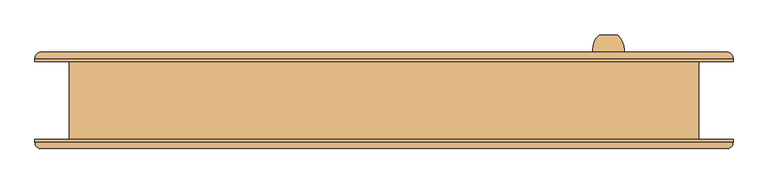
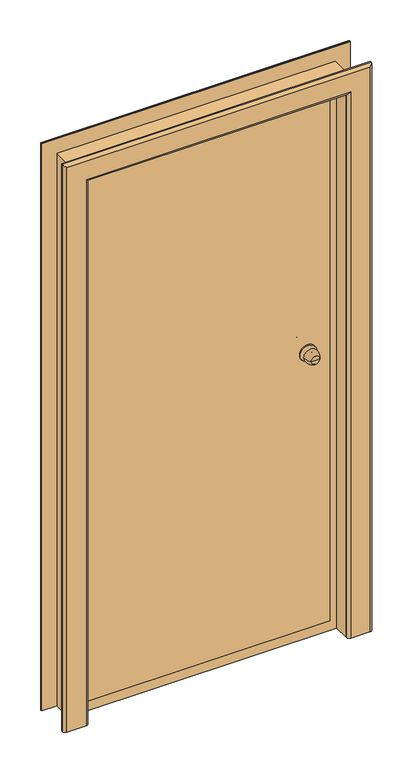
"""IFC4 building model written with IfcOpenShell, lengths in millimetres: door geometry, Наружная дверь 1-Навесная - Один проем наружу с порогом - 31173-2003 : ДСН КЛН  М1 УЗ 2100-1010 ГОСТ 31173-2003."""

import ifcopenshell
import ifcopenshell.guid

model = None  # the IFC model being written
_history = None  # IfcOwnerHistory: only IFC2X3 demands one
_inside = {}  # id of a spatial element -> (the spatial element, [elements in it])
_under = {}  # id of a project, library or spatial element -> (it, [spatial elements below it])
_declared = {}  # id of a project -> (the project, [libraries it declares])
_typed = {}  # id of a type object -> (the type object, [elements of that type])
_made_of = {}  # id of a material, layer set ... -> (it, [elements and type objects made of it])


def new_model(schema):
    """Start an empty IFC model of exactly this schema.

    Asked for "IFC4X3", IfcOpenShell would pick the latest addendum, in which some entities
    have other attributes; the version numbers below select the first issue.
    IFC2X3 requires an IfcOwnerHistory on every rooted entity: one is made here for all.
    """
    global model, _history
    if schema == "IFC4X3":
        model = ifcopenshell.file(schema_version=(4, 3, 0, 0))
    else:
        model = ifcopenshell.file(schema=schema)
    _inside.clear()
    _under.clear()
    _declared.clear()
    _typed.clear()
    _made_of.clear()
    _history = None
    if model.schema == "IFC2X3":
        org = make("IfcOrganization", Name="unknown")
        user = make(
            "IfcPersonAndOrganization",
            ThePerson=make("IfcPerson", FamilyName="unknown"),
            TheOrganization=org,
        )
        app = make(
            "IfcApplication",
            ApplicationDeveloper=org,
            Version="unknown",
            ApplicationFullName="unknown",
            ApplicationIdentifier="unknown",
        )
        _history = make(
            "IfcOwnerHistory",
            OwningUser=user,
            OwningApplication=app,
            ChangeAction="ADDED",
            CreationDate=0,
        )
    return model


def make(cls, **values):
    """One entity of the class cls with the attributes given. An attribute that is None is left unset."""
    return model.create_entity(
        cls, **{name: value for name, value in values.items() if value is not None}
    )


def rooted(cls, **values):
    """An entity with a GlobalId (a new one), such as an element, a storey or a relation."""
    return make(cls, GlobalId=ifcopenshell.guid.new(), OwnerHistory=_history, **values)


def si_unit(unit_type, name, prefix=None):
    """IfcSIUnit, for example si_unit("LENGTHUNIT", "METRE", prefix="MILLI")."""
    return make("IfcSIUnit", UnitType=unit_type, Prefix=prefix, Name=name)


def assignment(units):
    """IfcUnitAssignment: the units of a project."""
    return None if units is None else make("IfcUnitAssignment", Units=units)


def point(xyz):
    """IfcCartesianPoint."""
    return None if xyz is None else make("IfcCartesianPoint", Coordinates=xyz)


def direction(xyz):
    """IfcDirection."""
    return None if xyz is None else make("IfcDirection", DirectionRatios=xyz)


def frame(location, z_axis=None, x_axis=None):
    """IfcAxis2Placement3D, a coordinate frame: its origin and axes. An axis left out is left unset."""
    return make(
        "IfcAxis2Placement3D",
        Location=point(location),
        Axis=direction(z_axis),
        RefDirection=direction(x_axis),
    )


def origin():
    """The frame at (0, 0, 0) with its axes left unset."""
    return frame((0.0, 0.0, 0.0))


def place(relative_to, where):
    """IfcLocalPlacement: puts the frame where relative to a parent placement (None: the world)."""
    return make(
        "IfcLocalPlacement", PlacementRelTo=relative_to, RelativePlacement=where
    )


def context(
    kind, dimensions, precision=None, world=None, true_north=None, identifier=None
):
    """IfcGeometricRepresentationContext, for example the 3D "Model" context."""
    return make(
        "IfcGeometricRepresentationContext",
        ContextIdentifier=identifier,
        ContextType=kind,
        CoordinateSpaceDimension=dimensions,
        Precision=precision,
        WorldCoordinateSystem=world,
        TrueNorth=true_north,
    )


def project(units=None, contexts=None):
    """IfcProject with its units and contexts."""
    return rooted(
        "IfcProject",
        Name="project",
        RepresentationContexts=contexts,
        UnitsInContext=assignment(units),
    )


def spatial(cls, under=None, at=None, **own):
    """A site, building, storey or space (cls), placed at a placement, below another one or the project."""
    s = rooted(cls, ObjectPlacement=at, **own)
    if under is not None:
        _under.setdefault(under.id(), (under, []))[1].append(s)
    return s


def polyline(points):
    """IfcPolyline through the points."""
    return make("IfcPolyline", Points=[point(p) for p in points])


def circle_curve(where, radius):
    """IfcCircle in the frame where."""
    return make("IfcCircle", Position=where, Radius=radius)


def ellipse_curve(where, semi_axis1, semi_axis2):
    """IfcEllipse in the frame where."""
    return make(
        "IfcEllipse", Position=where, SemiAxis1=semi_axis1, SemiAxis2=semi_axis2
    )


def trimmed(basis, trim1, trim2, sense, master):
    """IfcTrimmedCurve: the piece of a basis curve between two trims."""
    return make(
        "IfcTrimmedCurve",
        BasisCurve=basis,
        Trim1=trim1,
        Trim2=trim2,
        SenseAgreement=sense,
        MasterRepresentation=master,
    )


def outline(outer, holes=None, kind="AREA"):
    """IfcArbitraryClosedProfileDef: a profile drawn as a closed curve; with holes, ...WithVoids."""
    if holes is None:
        return make("IfcArbitraryClosedProfileDef", ProfileType=kind, OuterCurve=outer)
    return make(
        "IfcArbitraryProfileDefWithVoids",
        ProfileType=kind,
        OuterCurve=outer,
        InnerCurves=holes,
    )


def extrude(swept, where, along, depth):
    """IfcExtrudedAreaSolid: the profile swept, set in the frame where, extruded along a direction by depth."""
    return make(
        "IfcExtrudedAreaSolid",
        SweptArea=swept,
        Position=where,
        ExtrudedDirection=direction(along),
        Depth=depth,
    )


def faces_of(points, faces, orient=None, outer=None):
    """IfcFace entities. A face is a list of loops; a loop is a list of indices into points, from 0.

    orient and outer hold one flag for each loop. By default every Orientation is true, the
    first loop of a face is its IfcFaceOuterBound and the others are IfcFaceBound.
    """
    made = []
    for i, loops in enumerate(faces):
        bounds = []
        for j, loop in enumerate(loops):
            is_outer = j == 0 if outer is None else outer[i][j]
            bounds.append(
                make(
                    "IfcFaceOuterBound" if is_outer else "IfcFaceBound",
                    Bound=make("IfcPolyLoop", Polygon=[points[k] for k in loop]),
                    Orientation=True if orient is None else orient[i][j],
                )
            )
        made.append(make("IfcFace", Bounds=bounds))
    return made


def faceted_brep(points, faces, orient=None, outer=None, voids=None):
    """IfcFacetedBrep: a solid bounded by flat faces; with voids (closed shells), ...WithVoids."""
    shared = [point(p) for p in points]
    hull = make("IfcClosedShell", CfsFaces=faces_of(shared, faces, orient, outer))
    if voids is None:
        return make("IfcFacetedBrep", Outer=hull)
    return make(
        "IfcFacetedBrepWithVoids",
        Outer=hull,
        Voids=[
            make(cls, CfsFaces=faces_of(shared, fs, o, b)) for cls, fs, o, b in voids
        ],
    )


def shape(context_of_items, identifier, shape_type, items):
    """IfcShapeRepresentation: the items that make up one representation, for example the "Body"."""
    return make(
        "IfcShapeRepresentation",
        ContextOfItems=context_of_items,
        RepresentationIdentifier=identifier,
        RepresentationType=shape_type,
        Items=items,
    )


def source(mapping_origin, context_of_items, identifier, shape_type, items):
    """IfcRepresentationMap: a shape defined once, which mapped items show again and again."""
    return make(
        "IfcRepresentationMap",
        MappingOrigin=mapping_origin,
        MappedRepresentation=shape(context_of_items, identifier, shape_type, items),
    )


def transform(
    local_origin,
    x_axis=None,
    y_axis=None,
    z_axis=None,
    scale=None,
    scale2=None,
    scale3=None,
    uniform=True,
):
    """IfcCartesianTransformationOperator3D, or its non-uniform kind. x_axis, y_axis, z_axis: its Axis1, 2, 3."""
    if uniform:
        return make(
            "IfcCartesianTransformationOperator3D",
            Axis1=direction(x_axis),
            Axis2=direction(y_axis),
            LocalOrigin=point(local_origin),
            Scale=scale,
            Axis3=direction(z_axis),
        )
    return make(
        "IfcCartesianTransformationOperator3DnonUniform",
        Axis1=direction(x_axis),
        Axis2=direction(y_axis),
        LocalOrigin=point(local_origin),
        Scale=scale,
        Axis3=direction(z_axis),
        Scale2=scale2,
        Scale3=scale3,
    )


def mapped(mapping_source, mapping_target):
    """IfcMappedItem: shows the shape of a source again, moved by a transform."""
    return make(
        "IfcMappedItem", MappingSource=mapping_source, MappingTarget=mapping_target
    )


def made_of(thing, what):
    """Note that an element or type object is made of a material, layer set ...; save() writes the relation."""
    if what is not None:
        _made_of.setdefault(what.id(), (what, []))[1].append(thing)
    return thing


def element(
    cls,
    number,
    at=None,
    inside=None,
    cuts=None,
    type_object=None,
    material=None,
    context=None,
    identifier="Body",
    shape_type=None,
    held_by="IfcProductDefinitionShape",
    body=None,
    shapes=None,
    **own,
):
    """One element of the class cls, such as IfcWall. Its Tag is "e" and its number.

    at: its placement. inside: the storey or other place that contains it. cuts: it is an
    opening in that element (IfcRelVoidsElement). A single representation is given by context,
    identifier, shape_type and body (its items); several are given by shapes. held_by: the class
    of the entity that holds the representations. save() writes the other relations.
    """
    e = rooted(cls, Tag="e%d" % number, ObjectPlacement=at, **own)
    if body is not None:
        shapes = [shape(context, identifier, shape_type, body)]
    if shapes is not None:
        e.Representation = make(held_by, Representations=shapes)
    if inside is not None:
        _inside.setdefault(inside.id(), (inside, []))[1].append(e)
    if cuts is not None:
        rooted(
            "IfcRelVoidsElement", RelatingBuildingElement=cuts, RelatedOpeningElement=e
        )
    if type_object is not None:
        _typed.setdefault(type_object.id(), (type_object, []))[1].append(e)
    return made_of(e, material)


def aggregate(whole, parts):
    """IfcRelAggregates: a whole, such as a stair, and the parts it consists of."""
    return rooted("IfcRelAggregates", RelatingObject=whole, RelatedObjects=parts)


def save(model, path):
    """Write the relations noted so far, then the file.

    IfcRelAggregates (storeys below a building ...), IfcRelContainedInSpatialStructure (elements
    in a storey), IfcRelDefinesByType, IfcRelAssociatesMaterial and IfcRelDeclares: one each for
    every whole, place, type object, material and project.
    """
    for whole, parts in _under.values():
        aggregate(whole, parts)
    for where, things in _inside.values():
        rooted(
            "IfcRelContainedInSpatialStructure",
            RelatedElements=things,
            RelatingStructure=where,
        )
    for kind, things in _typed.values():
        rooted("IfcRelDefinesByType", RelatedObjects=things, RelatingType=kind)
    for what, things in _made_of.values():
        rooted("IfcRelAssociatesMaterial", RelatedObjects=things, RelatingMaterial=what)
    for by, libraries in _declared.values():
        rooted("IfcRelDeclares", RelatingContext=by, RelatedDefinitions=libraries)
    model.write(path)


def plane_surface(at):
    """IfcPlane: the flat surface through the origin of the frame at, square to its z axis."""
    return make("IfcPlane", Position=at)


def cylinder_surface(at, radius):
    """IfcCylindricalSurface: all points at the distance radius from the z axis of the frame at."""
    return make("IfcCylindricalSurface", Position=at, Radius=radius)


def revolved_surface(curve, axis_point, axis_direction):
    """IfcSurfaceOfRevolution: the curve turned about the line through axis_point along axis_direction."""
    return make(
        "IfcSurfaceOfRevolution",
        SweptCurve=make("IfcArbitraryOpenProfileDef", ProfileType="CURVE", Curve=curve),
        AxisPosition=make("IfcAxis1Placement", Location=point(axis_point), Axis=direction(axis_direction)),
    )


def advanced_brep(points, edges, surfaces, faces):
    """IfcAdvancedBrep: a solid bounded by faces that lie on surfaces and meet in shared edges.

    An edge is (start, end): straight between two places in points (the first is 0);
    or (start, end, curve); or (start, end, curve, False) where it runs against its curve.
    A face is (place in surfaces, loops), or (place, loops, False) where it looks against
    its surface's normal. A loop lists edges by number (the first is 1), with a minus sign
    where the edge is run from its end to its start. The first loop is the outer one.
    """
    corners = [point(p) for p in points]
    vertices = [make("IfcVertexPoint", VertexGeometry=c) for c in corners]
    made = []
    for start, end, *more in edges:
        made.append(
            make(
                "IfcEdgeCurve",
                EdgeStart=vertices[start],
                EdgeEnd=vertices[end],
                EdgeGeometry=more[0] if more else make("IfcPolyline", Points=[corners[start], corners[end]]),
                SameSense=more[1] if len(more) > 1 else True,
            )
        )
    hull = []
    for where, loops, *sense in faces:
        bounds = []
        for j, loop in enumerate(loops):
            ring = [make("IfcOrientedEdge", EdgeElement=made[abs(k) - 1], Orientation=k > 0) for k in loop]
            bounds.append(
                make(
                    "IfcFaceOuterBound" if j == 0 else "IfcFaceBound",
                    Bound=make("IfcEdgeLoop", EdgeList=ring),
                    Orientation=True,
                )
            )
        hull.append(make("IfcAdvancedFace", Bounds=bounds, FaceSurface=surfaces[where], SameSense=sense[0] if sense else True))
    return make("IfcAdvancedBrep", Outer=make("IfcClosedShell", CfsFaces=hull))


def door_5ac3ea5e(model_context):
    return source(origin(), model_context, "Body", "SolidModel", [
        advanced_brep(
        [(345.0, 105.5, 1100.0), (375.0, 105.5, 1100.0), (360.0, 105.5, 1100.0), (335.0, 75.5, 1100.0), (385.0, 75.5, 1100.0), (342.0, 75.5, 1100.0), (378.0, 75.5, 1100.0), (350.0, 67.5, 1100.0), (370.0, 67.5, 1100.0), (350.0, 61.5, 1100.0), (370.0, 61.5, 1100.0), (390.0, 61.5, 1100.0), (330.0, 61.5, 1100.0), (390.0, 55.5, 1100.0), (330.0, 55.5, 1100.0)],
        [
            (0, 1, circle_curve(frame((360.0, 105.5, 1100.0), z_axis=(0.0, 1.0, 0.0), x_axis=(1.0, 0.0, 0.0)), 15.0)),
            (1, 2),
            (2, 0),
            (1, 0, circle_curve(frame((360.0, 105.5, 1100.0), z_axis=(0.0, 1.0, 0.0), x_axis=(1.0, 0.0, 0.0)), 15.0)),
            (0, 3, circle_curve(frame((369.6226265, 80.6257912, 1100.0), z_axis=(0.0, 0.0, 1.0), x_axis=(1.0, 0.0, 0.0)), 35.0)),
            (3, 4, circle_curve(frame((360.0, 75.5, 1100.0), z_axis=(0.0, 1.0, 0.0), x_axis=(1.0, 0.0, 0.0)), 25.0)),
            (4, 1, circle_curve(frame((350.3773735, 80.6257912, 1100.0), z_axis=(0.0, 0.0, 1.0), x_axis=(-1.0, 0.0, 0.0)), 35.0)),
            (4, 3, circle_curve(frame((360.0, 75.5, 1100.0), z_axis=(0.0, 1.0, 0.0), x_axis=(1.0, 0.0, 0.0)), 25.0)),
            (3, 5),
            (5, 6, circle_curve(frame((360.0, 75.5, 1100.0), z_axis=(0.0, 1.0, 0.0), x_axis=(1.0, 0.0, 0.0)), 18.0)),
            (6, 4),
            (6, 5, circle_curve(frame((360.0, 75.5, 1100.0), z_axis=(0.0, 1.0, 0.0), x_axis=(1.0, 0.0, 0.0)), 18.0)),
            (5, 7, circle_curve(frame((342.0, 67.5, 1100.0), z_axis=(0.0, 0.0, -1.0), x_axis=(1.0, 0.0, 0.0)), 8.0)),
            (7, 8, circle_curve(frame((360.0, 67.5, 1100.0), z_axis=(0.0, 1.0, 0.0), x_axis=(1.0, 0.0, 0.0)), 10.0)),
            (8, 6, circle_curve(frame((378.0, 67.5, 1100.0), z_axis=(0.0, 0.0, -1.0), x_axis=(-1.0, 0.0, 0.0)), 8.0)),
            (8, 7, circle_curve(frame((360.0, 67.5, 1100.0), z_axis=(0.0, 1.0, 0.0), x_axis=(1.0, 0.0, 0.0)), 10.0)),
            (7, 9),
            (9, 10, circle_curve(frame((360.0, 61.5, 1100.0), z_axis=(0.0, 1.0, 0.0), x_axis=(1.0, 0.0, 0.0)), 10.0)),
            (10, 8),
            (10, 9, circle_curve(frame((360.0, 61.5, 1100.0), z_axis=(0.0, 1.0, 0.0), x_axis=(1.0, 0.0, 0.0)), 10.0)),
            (11, 12, circle_curve(frame((360.0, 61.5, 1100.0), z_axis=(0.0, 1.0, 0.0), x_axis=(-1.0, 0.0, 0.0)), 30.0)),
            (12, 11, circle_curve(frame((360.0, 61.5, 1100.0), z_axis=(0.0, 1.0, 0.0), x_axis=(-1.0, 0.0, 0.0)), 30.0)),
            (13, 14, circle_curve(frame((360.0, 55.5, 1100.0), z_axis=(0.0, -1.0, 0.0), x_axis=(-1.0, 0.0, 0.0)), 30.0)),
            (14, 13, circle_curve(frame((360.0, 55.5, 1100.0), z_axis=(0.0, -1.0, 0.0), x_axis=(-1.0, 0.0, 0.0)), 30.0)),
            (11, 13),
            (14, 12),
        ],
        [
            plane_surface(frame((360.0, 105.5, 1100.0), z_axis=(0.0, 1.0, 0.0), x_axis=(1.0, 0.0, 0.0))),
            revolved_surface(trimmed(ellipse_curve(frame((350.3773735, 80.6257912, 1100.0), z_axis=(0.0, 0.0, -1.0), x_axis=(-1.0, 0.0, 0.0)), 35.0, 35.0), [point((375.0, 105.5, 1100.0))], [point((385.0, 75.5, 1100.0))], True, "CARTESIAN"), (360.0, 135.5, 1100.0), (0.0, -1.0, 0.0)),
            plane_surface(frame((360.0, 75.5, 1100.0), z_axis=(0.0, -1.0, 0.0), x_axis=(1.0, 0.0, 0.0))),
            revolved_surface(trimmed(ellipse_curve(frame((378.0, 67.5, 1100.0), z_axis=(0.0, 0.0, 1.0), x_axis=(-1.0, 0.0, 0.0)), 8.0, 8.0), [point((378.0, 75.5, 1100.0))], [point((370.0, 67.5, 1100.0))], True, "CARTESIAN"), (360.0, 135.5, 1100.0), (0.0, -1.0, 0.0)),
            cylinder_surface(frame((360.0, 135.5, 1100.0), z_axis=(0.0, -1.0, 0.0), x_axis=(1.0, 0.0, 0.0)), 10.0),
            plane_surface(frame((330.0, 61.5, 1100.0), z_axis=(0.0, 1.0, 0.0), x_axis=(0.0, 0.0, 1.0))),
            plane_surface(frame((330.0, 55.5, 1100.0), z_axis=(0.0, -1.0, 0.0), x_axis=(0.0, 0.0, -1.0))),
            cylinder_surface(frame((360.0, 55.5, 1100.0), z_axis=(0.0, 1.0, 0.0), x_axis=(-1.0, 0.0, 0.0)), 30.0),
        ],
        [
            (0, [[1, 2, 3]]),
            (0, [[-2, 4, -3]]),
            (1, [[-1, 5, 6, 7]]),
            (1, [[-4, -7, 8, -5]]),
            (2, [[-6, 9, 10, 11]]),
            (2, [[-8, -11, 12, -9]]),
            (3, [[-10, 13, 14, 15]]),
            (3, [[-12, -15, 16, -13]]),
            (4, [[-14, 17, 18, 19]]),
            (4, [[-16, -19, 20, -17]]),
            (5, [[21, 22], [-18, -20]]),
            (6, [[23, 24]]),
            (7, [[-21, 25, -24, 26]]),
            (7, [[-22, -26, -23, -25]]),
        ],
    ),
        advanced_brep(
        [(375.0, -64.5, 1100.0), (345.0, -64.5, 1100.0), (360.0, -64.5, 1100.0), (385.0, -34.5, 1100.0), (335.0, -34.5, 1100.0), (378.0, -34.5, 1100.0), (342.0, -34.5, 1100.0), (370.0, -26.5, 1100.0), (350.0, -26.5, 1100.0), (370.0, -20.5, 1100.0), (350.0, -20.5, 1100.0), (330.0, -20.5, 1100.0), (390.0, -20.5, 1100.0), (330.0, -14.5, 1100.0), (390.0, -14.5, 1100.0)],
        [
            (0, 1, circle_curve(frame((360.0, -64.5, 1100.0), z_axis=(0.0, -1.0, 0.0), x_axis=(-1.0, 0.0, 0.0)), 15.0)),
            (1, 2),
            (2, 0),
            (1, 0, circle_curve(frame((360.0, -64.5, 1100.0), z_axis=(0.0, -1.0, 0.0), x_axis=(-1.0, 0.0, 0.0)), 15.0)),
            (0, 3, circle_curve(frame((350.3773735, -39.6257912, 1100.0), z_axis=(0.0, 0.0, 1.0), x_axis=(-1.0, 0.0, 0.0)), 35.0)),
            (3, 4, circle_curve(frame((360.0, -34.5, 1100.0), z_axis=(0.0, -1.0, 0.0), x_axis=(-1.0, 0.0, 0.0)), 25.0)),
            (4, 1, circle_curve(frame((369.6226265, -39.6257912, 1100.0), z_axis=(0.0, 0.0, 1.0), x_axis=(1.0, 0.0, 0.0)), 35.0)),
            (4, 3, circle_curve(frame((360.0, -34.5, 1100.0), z_axis=(0.0, -1.0, 0.0), x_axis=(-1.0, 0.0, 0.0)), 25.0)),
            (3, 5),
            (5, 6, circle_curve(frame((360.0, -34.5, 1100.0), z_axis=(0.0, -1.0, 0.0), x_axis=(-1.0, 0.0, 0.0)), 18.0)),
            (6, 4),
            (6, 5, circle_curve(frame((360.0, -34.5, 1100.0), z_axis=(0.0, -1.0, 0.0), x_axis=(-1.0, 0.0, 0.0)), 18.0)),
            (5, 7, circle_curve(frame((378.0, -26.5, 1100.0), z_axis=(0.0, 0.0, -1.0), x_axis=(-1.0, 0.0, 0.0)), 8.0)),
            (7, 8, circle_curve(frame((360.0, -26.5, 1100.0), z_axis=(0.0, -1.0, 0.0), x_axis=(-1.0, 0.0, 0.0)), 10.0)),
            (8, 6, circle_curve(frame((342.0, -26.5, 1100.0), z_axis=(0.0, 0.0, -1.0), x_axis=(1.0, 0.0, 0.0)), 8.0)),
            (8, 7, circle_curve(frame((360.0, -26.5, 1100.0), z_axis=(0.0, -1.0, 0.0), x_axis=(-1.0, 0.0, 0.0)), 10.0)),
            (7, 9),
            (9, 10, circle_curve(frame((360.0, -20.5, 1100.0), z_axis=(0.0, -1.0, 0.0), x_axis=(-1.0, 0.0, 0.0)), 10.0)),
            (10, 8),
            (10, 9, circle_curve(frame((360.0, -20.5, 1100.0), z_axis=(0.0, -1.0, 0.0), x_axis=(-1.0, 0.0, 0.0)), 10.0)),
            (11, 12, circle_curve(frame((360.0, -20.5, 1100.0), z_axis=(0.0, -1.0, 0.0), x_axis=(1.0, 0.0, 0.0)), 30.0)),
            (12, 11, circle_curve(frame((360.0, -20.5, 1100.0), z_axis=(0.0, -1.0, 0.0), x_axis=(1.0, 0.0, 0.0)), 30.0)),
            (13, 14, circle_curve(frame((360.0, -14.5, 1100.0), z_axis=(0.0, 1.0, 0.0), x_axis=(1.0, 0.0, 0.0)), 30.0)),
            (14, 13, circle_curve(frame((360.0, -14.5, 1100.0), z_axis=(0.0, 1.0, 0.0), x_axis=(1.0, 0.0, 0.0)), 30.0)),
            (11, 13),
            (14, 12),
        ],
        [
            plane_surface(frame((360.0, -64.5, 1100.0), z_axis=(0.0, -1.0, 0.0), x_axis=(-1.0, 0.0, 0.0))),
            revolved_surface(trimmed(ellipse_curve(frame((369.6226265, -39.6257912, 1100.0), z_axis=(0.0, 0.0, -1.0), x_axis=(1.0, 0.0, 0.0)), 35.0, 35.0), [point((345.0, -64.5, 1100.0))], [point((335.0, -34.5, 1100.0))], True, "CARTESIAN"), (360.0, -94.5, 1100.0), (0.0, 1.0, 0.0)),
            plane_surface(frame((360.0, -34.5, 1100.0), z_axis=(0.0, 1.0, 0.0), x_axis=(-1.0, 0.0, 0.0))),
            revolved_surface(trimmed(ellipse_curve(frame((342.0, -26.5, 1100.0), z_axis=(0.0, 0.0, 1.0), x_axis=(1.0, 0.0, 0.0)), 8.0, 8.0), [point((342.0, -34.5, 1100.0))], [point((350.0, -26.5, 1100.0))], True, "CARTESIAN"), (360.0, -94.5, 1100.0), (0.0, 1.0, 0.0)),
            cylinder_surface(frame((360.0, -94.5, 1100.0), z_axis=(0.0, 1.0, 0.0), x_axis=(-1.0, 0.0, 0.0)), 10.0),
            plane_surface(frame((390.0, -20.5, 1100.0), z_axis=(0.0, -1.0, 0.0), x_axis=(0.0, 0.0, 1.0))),
            plane_surface(frame((390.0, -14.5, 1100.0), z_axis=(0.0, 1.0, 0.0), x_axis=(0.0, 0.0, -1.0))),
            cylinder_surface(frame((360.0, -14.5, 1100.0), z_axis=(0.0, -1.0, 0.0), x_axis=(1.0, 0.0, 0.0)), 30.0),
        ],
        [
            (0, [[1, 2, 3]]),
            (0, [[-2, 4, -3]]),
            (1, [[-1, 5, 6, 7]]),
            (1, [[-4, -7, 8, -5]]),
            (2, [[-6, 9, 10, 11]]),
            (2, [[-8, -11, 12, -9]]),
            (3, [[-10, 13, 14, 15]]),
            (3, [[-12, -15, 16, -13]]),
            (4, [[-14, 17, 18, 19]]),
            (4, [[-16, -19, 20, -17]]),
            (5, [[21, 22], [-18, -20]]),
            (6, [[23, 24]]),
            (7, [[-21, 25, -24, 26]]),
            (7, [[-22, -26, -23, -25]]),
        ],
    ),
        faceted_brep([(440.0, -14.5, 42.0), (-440.0, -14.5, 42.0), (-440.0, -9.5, 42.0), (440.0, -9.5, 42.0), (440.0, -14.5, 2055.0), (440.0, -9.5, 2055.0), (-440.0, -9.5, 2055.0), (420.0, -9.5, 2035.0), (-420.0, -9.5, 2035.0), (-420.0, -9.5, 62.0), (420.0, -9.5, 62.0), (-440.0, -14.5, 2055.0), (420.0, 55.5, 62.0), (420.0, 55.5, 2035.0), (-420.0, 55.5, 62.0), (-420.0, 55.5, 2035.0)], [[[0, 1, 2, 3]], [[4, 0, 3, 5]], [[5, 3, 2, 6], [7, 8, 9, 10]], [[2, 1, 11, 6]], [[11, 1, 0, 4]], [[7, 10, 12, 13]], [[9, 14, 12, 10]], [[15, 14, 9, 8]], [[13, 12, 14, 15]], [[4, 5, 6, 11]], [[7, 13, 15, 8]]]),
        extrude(outline(polyline([(0.0, 485.0), (2100.0, 485.0), (2100.0, -485.0), (0.0, -485.0), (0.0, -470.0), (2085.0, -470.0), (2085.0, 470.0), (0.0, 470.0), (0.0, 485.0)])), frame((0.0, -62.5, 0.0), z_axis=(0.0, 1.0, 0.0), x_axis=(0.0, 0.0, 1.0)), (0.0, 0.0, 1.0), 55.0),
        faceted_brep([(485.0, -7.5, 0.0), (-485.0, -7.5, 0.0), (-485.0, 62.5, 0.0), (485.0, 62.5, 0.0), (-485.0, -7.5, 2100.0), (-485.0, 62.5, 2100.0), (485.0, 62.5, 2100.0), (-405.0, 62.5, 2020.0), (-405.0, 62.5, 80.0), (405.0, 62.5, 80.0), (405.0, 62.5, 2020.0), (485.0, -7.5, 2100.0), (-425.0, -7.5, 60.0), (-425.0, -7.5, 2040.0), (425.0, -7.5, 2040.0), (425.0, -7.5, 60.0), (425.0, 57.5, 60.0), (-425.0, 57.5, 60.0), (-425.0, 57.5, 2040.0), (425.0, 57.5, 2040.0), (-405.0, 57.5, 80.0), (-405.0, 57.5, 2020.0), (405.0, 57.5, 2020.0), (405.0, 57.5, 80.0)], [[[0, 1, 2, 3]], [[1, 4, 5, 2]], [[2, 5, 6, 3], [7, 8, 9, 10]], [[4, 1, 0, 11], [12, 13, 14, 15]], [[16, 17, 12, 15]], [[17, 18, 13, 12]], [[18, 17, 16, 19], [20, 21, 22, 23]], [[9, 8, 20, 23]], [[8, 7, 21, 20]], [[11, 0, 3, 6]], [[19, 16, 15, 14]], [[10, 9, 23, 22]], [[4, 11, 6, 5]], [[18, 19, 14, 13]], [[7, 10, 22, 21]]]),
        advanced_brep(
        [(-560.0, 62.5, 0.0), (-560.0, 67.5, 0.0), (-550.0, 77.5, 0.0), (-480.0, 77.5, 0.0), (-470.0, 67.5, 0.0), (-470.0, 62.5, 0.0), (-470.0, 62.5, 2085.0), (470.0, 62.5, 2085.0), (470.0, 62.5, 0.0), (560.0, 62.5, 0.0), (560.0, 62.5, 2175.0), (-560.0, 62.5, 2175.0), (-470.0, 67.5, 2085.0), (-480.0, 77.5, 2095.0), (-550.0, 77.5, 2165.0), (550.0, 77.5, 2165.0), (550.0, 77.5, 0.0), (480.0, 77.5, 0.0), (480.0, 77.5, 2095.0), (-560.0, 67.5, 2175.0), (560.0, 67.5, 0.0), (560.0, 67.5, 2175.0), (470.0, 67.5, 0.0), (470.0, 67.5, 2085.0)],
        [
            (0, 1),
            (1, 2, circle_curve(frame((-550.0, 67.5, 0.0), z_axis=(0.0, 0.0, -1.0), x_axis=(-1.0, 0.0, 0.0)), 10.0)),
            (2, 3),
            (3, 4, circle_curve(frame((-480.0, 67.5, 0.0), z_axis=(0.0, 0.0, -1.0), x_axis=(-1.0, 0.0, 0.0)), 10.0)),
            (4, 5),
            (5, 0),
            (5, 6),
            (6, 7),
            (7, 8),
            (8, 9),
            (9, 10),
            (10, 11),
            (11, 0),
            (4, 12),
            (12, 6),
            (3, 13),
            (13, 12, ellipse_curve(frame((-480.0, 67.5, 2095.0), z_axis=(-0.7071067811865475, 0.0, -0.7071067811865475), x_axis=(0.7071067811865474, 0.0, -0.7071067811865476)), 14.1421356, 10.0)),
            (2, 14),
            (14, 15),
            (15, 16),
            (16, 17),
            (17, 18),
            (18, 13),
            (1, 19),
            (19, 14, ellipse_curve(frame((-550.0, 67.5, 2165.0), z_axis=(-0.7071067811865475, 0.0, -0.7071067811865475), x_axis=(0.7071067811865474, 0.0, -0.7071067811865476)), 14.1421356, 10.0)),
            (11, 19),
            (9, 20),
            (20, 21),
            (21, 10),
            (8, 22),
            (22, 17, circle_curve(frame((480.0, 67.5, 0.0), z_axis=(0.0, 0.0, -1.0), x_axis=(1.0, 0.0, 0.0)), 10.0)),
            (16, 20, circle_curve(frame((550.0, 67.5, 0.0), z_axis=(0.0, 0.0, -1.0), x_axis=(1.0, 0.0, 0.0)), 10.0)),
            (23, 22),
            (7, 23),
            (23, 18, ellipse_curve(frame((480.0, 67.5, 2095.0), z_axis=(0.7071067811865475, 0.0, -0.7071067811865475), x_axis=(0.7071067811865474, 0.0, 0.7071067811865476)), 14.1421356, 10.0)),
            (15, 21, ellipse_curve(frame((550.0, 67.5, 2165.0), z_axis=(0.7071067811865475, 0.0, -0.7071067811865475), x_axis=(0.7071067811865474, 0.0, 0.7071067811865476)), 14.1421356, 10.0)),
            (12, 23),
            (19, 21),
        ],
        [
            plane_surface(frame((-505.0, 62.5, 0.0), z_axis=(0.0, 0.0, -1.0), x_axis=(0.0, 1.0, 0.0))),
            plane_surface(frame((-560.0, 62.5, 0.0), z_axis=(0.0, -1.0, 0.0), x_axis=(0.0, 0.0, 1.0))),
            plane_surface(frame((-470.0, 62.5, 0.0), z_axis=(1.0, 0.0, 0.0), x_axis=(0.0, 0.0, 1.0))),
            cylinder_surface(frame((-480.0, 67.5, 0.0), z_axis=(0.0, 0.0, -1.0), x_axis=(-1.0, 0.0, 0.0)), 10.0),
            plane_surface(frame((-480.0, 77.5, 0.0), z_axis=(0.0, 1.0, 0.0), x_axis=(0.0, 0.0, 1.0))),
            cylinder_surface(frame((-550.0, 67.5, 0.0), z_axis=(0.0, 0.0, -1.0), x_axis=(-1.0, 0.0, 0.0)), 10.0),
            plane_surface(frame((-560.0, 67.5, 0.0), z_axis=(-1.0, 0.0, 0.0), x_axis=(0.0, 0.0, 1.0))),
            plane_surface(frame((560.0, 67.5, 2175.0), z_axis=(1.0, 0.0, 0.0), x_axis=(0.0, 0.0, -1.0))),
            plane_surface(frame((505.0, 62.5, 0.0), z_axis=(0.0, 0.0, -1.0), x_axis=(0.0, 1.0, 0.0))),
            plane_surface(frame((470.0, 62.5, 2085.0), z_axis=(-1.0, 0.0, 0.0), x_axis=(0.0, 0.0, -1.0))),
            cylinder_surface(frame((480.0, 67.5, 2120.0), z_axis=(0.0, 0.0, 1.0), x_axis=(1.0, 0.0, 0.0)), 10.0),
            cylinder_surface(frame((550.0, 67.5, 2120.0), z_axis=(0.0, 0.0, 1.0), x_axis=(1.0, 0.0, 0.0)), 10.0),
            plane_surface(frame((-470.0, 62.5, 2085.0), z_axis=(0.0, 0.0, -1.0), x_axis=(1.0, 0.0, 0.0))),
            cylinder_surface(frame((-505.0, 67.5, 2095.0), z_axis=(-1.0, 0.0, 0.0), x_axis=(0.0, 0.0, 1.0)), 10.0),
            cylinder_surface(frame((-505.0, 67.5, 2165.0), z_axis=(-1.0, 0.0, 0.0), x_axis=(0.0, 0.0, 1.0)), 10.0),
            plane_surface(frame((-560.0, 67.5, 2175.0), z_axis=(0.0, 0.0, 1.0), x_axis=(1.0, 0.0, 0.0))),
        ],
        [
            (0, [[1, 2, 3, 4, 5, 6]]),
            (1, [[7, 8, 9, 10, 11, 12, 13, -6]]),
            (2, [[14, 15, -7, -5]]),
            (3, [[16, 17, -14, -4]]),
            (4, [[18, 19, 20, 21, 22, 23, -16, -3]]),
            (5, [[24, 25, -18, -2]]),
            (6, [[-13, 26, -24, -1]]),
            (7, [[-11, 27, 28, 29]]),
            (8, [[-10, 30, 31, -21, 32, -27]]),
            (9, [[33, -30, -9, 34]]),
            (10, [[-22, -31, -33, 35]]),
            (11, [[-28, -32, -20, 36]]),
            (12, [[37, -34, -8, -15]]),
            (13, [[-23, -35, -37, -17]]),
            (14, [[38, -36, -19, -25]]),
            (15, [[-12, -29, -38, -26]]),
        ],
    ),
        advanced_brep(
        [(560.0, -62.5, 0.0), (560.0, -67.5, 0.0), (550.0, -77.5, 0.0), (480.0, -77.5, 0.0), (470.0, -67.5, 0.0), (470.0, -62.5, 0.0), (470.0, -62.5, 2085.0), (-470.0, -62.5, 2085.0), (-470.0, -62.5, 0.0), (-560.0, -62.5, 0.0), (-560.0, -62.5, 2175.0), (560.0, -62.5, 2175.0), (470.0, -67.5, 2085.0), (480.0, -77.5, 2095.0), (550.0, -77.5, 2165.0), (-550.0, -77.5, 2165.0), (-550.0, -77.5, 0.0), (-480.0, -77.5, 0.0), (-480.0, -77.5, 2095.0), (560.0, -67.5, 2175.0), (-560.0, -67.5, 0.0), (-560.0, -67.5, 2175.0), (-470.0, -67.5, 0.0), (-470.0, -67.5, 2085.0)],
        [
            (0, 1),
            (1, 2, circle_curve(frame((550.0, -67.5, 0.0), z_axis=(0.0, 0.0, -1.0), x_axis=(1.0, 0.0, 0.0)), 10.0)),
            (2, 3),
            (3, 4, circle_curve(frame((480.0, -67.5, 0.0), z_axis=(0.0, 0.0, -1.0), x_axis=(1.0, 0.0, 0.0)), 10.0)),
            (4, 5),
            (5, 0),
            (5, 6),
            (6, 7),
            (7, 8),
            (8, 9),
            (9, 10),
            (10, 11),
            (11, 0),
            (4, 12),
            (12, 6),
            (3, 13),
            (13, 12, ellipse_curve(frame((480.0, -67.5, 2095.0), z_axis=(0.7071067811865475, 0.0, -0.7071067811865475), x_axis=(-0.7071067811865474, 0.0, -0.7071067811865476)), 14.1421356, 10.0)),
            (2, 14),
            (14, 15),
            (15, 16),
            (16, 17),
            (17, 18),
            (18, 13),
            (1, 19),
            (19, 14, ellipse_curve(frame((550.0, -67.5, 2165.0), z_axis=(0.7071067811865475, 0.0, -0.7071067811865475), x_axis=(-0.7071067811865474, 0.0, -0.7071067811865476)), 14.1421356, 10.0)),
            (11, 19),
            (9, 20),
            (20, 21),
            (21, 10),
            (8, 22),
            (22, 17, circle_curve(frame((-480.0, -67.5, 0.0), z_axis=(0.0, 0.0, -1.0), x_axis=(-1.0, 0.0, 0.0)), 10.0)),
            (16, 20, circle_curve(frame((-550.0, -67.5, 0.0), z_axis=(0.0, 0.0, -1.0), x_axis=(-1.0, 0.0, 0.0)), 10.0)),
            (23, 22),
            (7, 23),
            (23, 18, ellipse_curve(frame((-480.0, -67.5, 2095.0), z_axis=(-0.7071067811865475, 0.0, -0.7071067811865475), x_axis=(-0.7071067811865474, 0.0, 0.7071067811865476)), 14.1421356, 10.0)),
            (15, 21, ellipse_curve(frame((-550.0, -67.5, 2165.0), z_axis=(-0.7071067811865475, 0.0, -0.7071067811865475), x_axis=(-0.7071067811865474, 0.0, 0.7071067811865476)), 14.1421356, 10.0)),
            (12, 23),
            (19, 21),
        ],
        [
            plane_surface(frame((505.0, -62.5, 0.0), z_axis=(0.0, 0.0, -1.0), x_axis=(0.0, 1.0, 0.0))),
            plane_surface(frame((560.0, -62.5, 0.0), z_axis=(0.0, 1.0, 0.0), x_axis=(0.0, 0.0, 1.0))),
            plane_surface(frame((470.0, -62.5, 0.0), z_axis=(-1.0, 0.0, 0.0), x_axis=(0.0, 0.0, 1.0))),
            cylinder_surface(frame((480.0, -67.5, 0.0), z_axis=(0.0, 0.0, -1.0), x_axis=(1.0, 0.0, 0.0)), 10.0),
            plane_surface(frame((480.0, -77.5, 0.0), z_axis=(0.0, -1.0, 0.0), x_axis=(0.0, 0.0, 1.0))),
            cylinder_surface(frame((550.0, -67.5, 0.0), z_axis=(0.0, 0.0, -1.0), x_axis=(1.0, 0.0, 0.0)), 10.0),
            plane_surface(frame((560.0, -67.5, 0.0), z_axis=(1.0, 0.0, 0.0), x_axis=(0.0, 0.0, 1.0))),
            plane_surface(frame((-560.0, -67.5, 2175.0), z_axis=(-1.0, 0.0, 0.0), x_axis=(0.0, 0.0, -1.0))),
            plane_surface(frame((-505.0, -62.5, 0.0), z_axis=(0.0, 0.0, -1.0), x_axis=(0.0, 1.0, 0.0))),
            plane_surface(frame((-470.0, -62.5, 2085.0), z_axis=(1.0, 0.0, 0.0), x_axis=(0.0, 0.0, -1.0))),
            cylinder_surface(frame((-480.0, -67.5, 2120.0), z_axis=(0.0, 0.0, 1.0), x_axis=(-1.0, 0.0, 0.0)), 10.0),
            cylinder_surface(frame((-550.0, -67.5, 2120.0), z_axis=(0.0, 0.0, 1.0), x_axis=(-1.0, 0.0, 0.0)), 10.0),
            plane_surface(frame((470.0, -62.5, 2085.0), z_axis=(0.0, 0.0, -1.0), x_axis=(-1.0, 0.0, 0.0))),
            cylinder_surface(frame((505.0, -67.5, 2095.0), z_axis=(1.0, 0.0, 0.0), x_axis=(0.0, 0.0, 1.0)), 10.0),
            cylinder_surface(frame((505.0, -67.5, 2165.0), z_axis=(1.0, 0.0, 0.0), x_axis=(0.0, 0.0, 1.0)), 10.0),
            plane_surface(frame((560.0, -67.5, 2175.0), z_axis=(0.0, 0.0, 1.0), x_axis=(-1.0, 0.0, 0.0))),
        ],
        [
            (0, [[1, 2, 3, 4, 5, 6]]),
            (1, [[7, 8, 9, 10, 11, 12, 13, -6]]),
            (2, [[14, 15, -7, -5]]),
            (3, [[16, 17, -14, -4]]),
            (4, [[18, 19, 20, 21, 22, 23, -16, -3]]),
            (5, [[24, 25, -18, -2]]),
            (6, [[-13, 26, -24, -1]]),
            (7, [[-11, 27, 28, 29]]),
            (8, [[-10, 30, 31, -21, 32, -27]]),
            (9, [[33, -30, -9, 34]]),
            (10, [[-22, -31, -33, 35]]),
            (11, [[-28, -32, -20, 36]]),
            (12, [[37, -34, -8, -15]]),
            (13, [[-23, -35, -37, -17]]),
            (14, [[38, -36, -19, -25]]),
            (15, [[-12, -29, -38, -26]]),
        ],
    ),
        extrude(outline(polyline([(0.0, 505.0), (2120.0, 505.0), (2120.0, -505.0), (0.0, -505.0), (0.0, -485.0), (2100.0, -485.0), (2100.0, 485.0), (0.0, 485.0), (0.0, 505.0)])), frame((0.0, -62.5, 0.0), z_axis=(0.0, 1.0, 0.0), x_axis=(0.0, 0.0, 1.0)), (0.0, 0.0, 1.0), 125.0),
    ])


if __name__ == "__main__":
    model = new_model("IFC4")
    model_context = context("Model", 3, world=origin())
    ifc_project = project(units=[si_unit("LENGTHUNIT", "METRE", prefix="MILLI")], contexts=[model_context])
    site = spatial("IfcSite", under=ifc_project)
    building = spatial("IfcBuilding", under=site)
    placement = place(None, origin())
    door_shape = door_5ac3ea5e(model_context)
    element("IfcDoor", 1, ObjectType="Наружная дверь 1-Навесная - Один проем наружу с порогом - 31173-2003 : ДСН КЛН  М1 УЗ 2100-1010 ГОСТ 31173-2003", at=placement, inside=building, context=model_context, shape_type="MappedRepresentation", body=[
        mapped(door_shape, transform((0.0, 0.0, 0.0), x_axis=(1.0, 0.0, 0.0), y_axis=(0.0, 1.0, 0.0), z_axis=(0.0, 0.0, 1.0))),
    ])
    save(model, "model.ifc")

# Revit data of these elements
# Type "Наружная дверь 1-Навесная - Один проем наружу с порогом - 31173-2003 : ДСН КЛН  М1 УЗ 2100-1010 ГОСТ 31173-2003"
#   Type Mark = "148"
#   Description = "ДСН КЛН  М1 УЗ 2100-900 ГОСТ 31173-2003"
#   Проекционное соединение по ширине = 90 mm
#   Rough Width = 1010 mm
#   Rough Height = 2120 mm
#   Угол проема [instance default] = 30°
#   Толщина_Тепл_Изоляции = 20 mm
#   Heat Transfer Coefficient (U) = 3.7021 W/(m²·K)
#   Height = 2100 mm
#   Width = 970 mm
#   Ширина каркаса = 60 mm
#   Толщина каркаса = 70 mm
#   Вставка двери [instance default] = 0 mm
#   Правая сторона = no
#   Левая сторона = yes
#   Function = 1
#   Обрезка = Сталь
#   Панель = Сталь
#   Тепловая изоляция = Тепловая изоляция
#   Кадр = Сталь
#   Дверная ручка = Металл
#   Visual Light Transmittance = 0
#   Solar Heat Gain Coefficient = 0
#   Construction Type Id = ""
#   Wall Closure = (empty or 0)
#   Analytic Construction = (empty or 0)
# Element 1 (IfcDoor, "Наружная дверь 1-Навесная - Один проем наружу с порогом - 31173-2003 : ДСН КЛН  М1 УЗ 2100-1010 ГОСТ 31173-2003")
#   Materials on its faces: "Сталь", "Металл", "Тепловая изоляция"
# Materials
#   "Сталь": class "Металл", colour RGB 247 247 247, transparency 0
#   "Тепловая изоляция": class "Пластмасса", colour RGB 185 154 119, transparency 0, Cost = 0
#   "Металл": class "Металл", colour RGB 249 249 249, transparency 0
